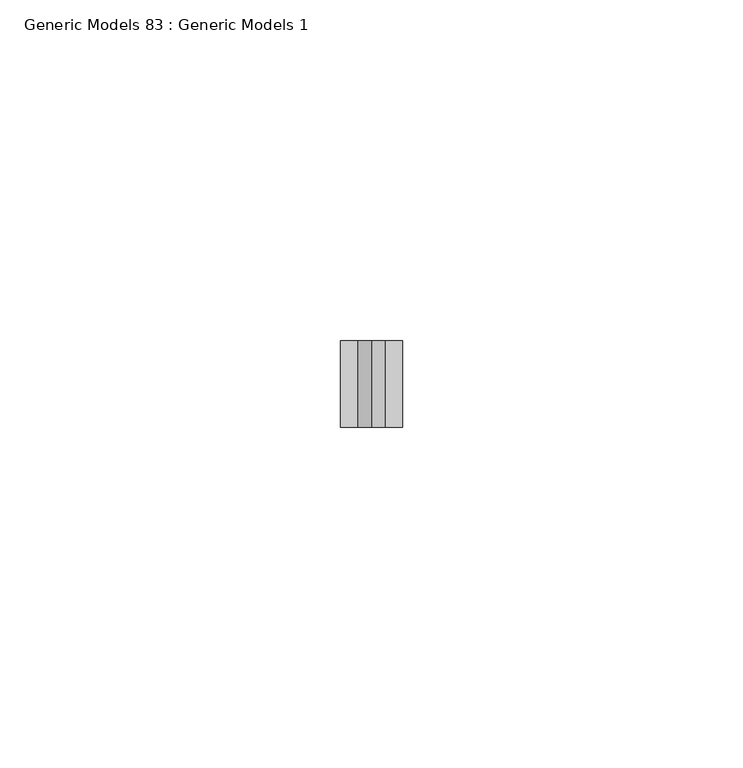
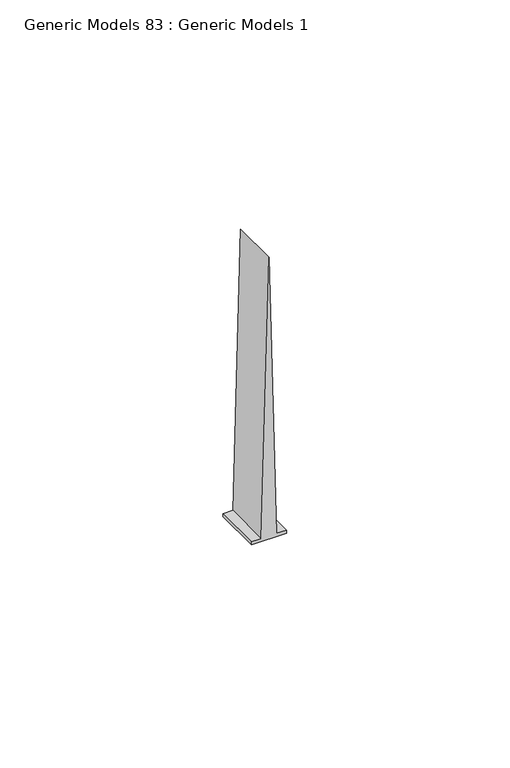
"""IFC4 building model written with IfcOpenShell, lengths in millimetres: proxy geometry, Generic Models 83 : Generic Models 1."""

from ifc_helpers import new_model, si_unit, frame, origin, place, context, project, spatial, polyline, outline, extrude, source, transform, mapped, element, save


def generic_models_83_generic_models_1_66a13d42(model_context):
    return source(origin(), model_context, "Body", "SweptSolid", [
        extrude(outline(polyline([(2457.6119589, 49845.474547), (2457.6119589, 49854.567747), (2458.4057089, 49854.567747), (2458.4057089, 49852.0178834), (2534.6057089, 49850.021147), (2458.4057089, 49848.0244106), (2458.4057089, 49845.474547), (2457.6119589, 49845.474547)])), frame((0.0, 565.15, 0.0), z_axis=(0.0, 1.0, 0.0), x_axis=(0.0, 0.0, 1.0)), (0.0, 0.0, 1.0), 12.7),
    ])


if __name__ == "__main__":
    model = new_model("IFC4")
    model_context = context("Model", 3, world=origin())
    ifc_project = project(units=[si_unit("LENGTHUNIT", "METRE", prefix="MILLI")], contexts=[model_context])
    site = spatial("IfcSite", under=ifc_project)
    building = spatial("IfcBuilding", under=site)
    placement = place(None, origin())
    generic_models_83_generic_models_1_shape = generic_models_83_generic_models_1_66a13d42(model_context)
    element("IfcBuildingElementProxy", 1, Name="Generic Models 83 : Generic Models 1", ObjectType="Generic Models 83 : Generic Models 1", at=placement, inside=building, context=model_context, shape_type="MappedRepresentation", body=[
        mapped(generic_models_83_generic_models_1_shape, transform((0.0, 0.0, 0.0), x_axis=(1.0, 0.0, 0.0), y_axis=(0.0, 1.0, 0.0), z_axis=(0.0, 0.0, 1.0))),
    ])
    save(model, "model.ifc")

# Revit data of these elements
# Element 1 (IfcBuildingElementProxy, "Generic Models 83 : Generic Models 1")
#   Materials on its faces: "ATTACH GYPSUM BOARD TO STUDS AND NOT TO TOP TRACK"
# Materials
#   "ATTACH GYPSUM BOARD TO STUDS AND NOT TO TOP TRACK": class "Generic", colour RGB 48 48 48, transparency 0, Cost = 0
